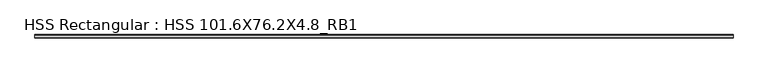
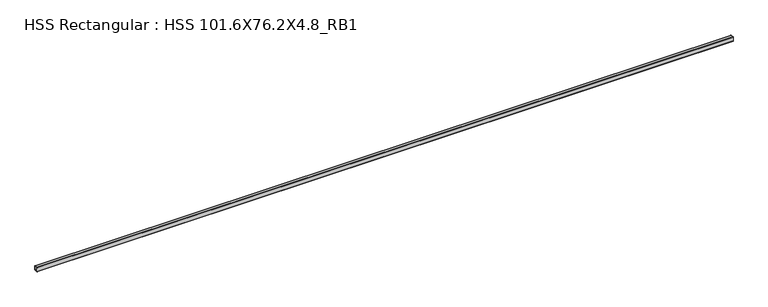
"""IFC4 building model written with IfcOpenShell, lengths in millimetres: beam geometry, HSS Rectangular : HSS 101.6X76.2X4.8_RB1."""

from ifc_helpers import new_model, si_unit, point, frame, frame_2d, origin, place, context, project, spatial, polyline, circle_curve, trimmed, segment, composite_curve, outline, extrude, source, transform, mapped, element, save


def hss_rectangular_hss_101_6x76_2x4_8_rb1_f7a6f8b3(model_context):
    return source(origin(), model_context, "Body", "SweptSolid", [
        extrude(outline(composite_curve([segment(trimmed(circle_curve(frame_2d((-28.575, 41.275)), 9.525), [point((-38.1, 41.275))], [point((-28.575, 50.8))], False, "CARTESIAN"), True, "CONTINUOUS"), segment(polyline([(-28.575, 50.8), (28.575, 50.8)]), True, "CONTINUOUS"), segment(trimmed(circle_curve(frame_2d((28.575, 41.275)), 9.525), [point((28.575, 50.8))], [point((38.1, 41.275))], False, "CARTESIAN"), True, "CONTINUOUS"), segment(polyline([(38.1, 41.275), (38.1, -41.275)]), True, "CONTINUOUS"), segment(trimmed(circle_curve(frame_2d((28.575, -41.275)), 9.525), [point((38.1, -41.275))], [point((28.575, -50.8))], False, "CARTESIAN"), True, "CONTINUOUS"), segment(polyline([(28.575, -50.8), (-28.575, -50.8)]), True, "CONTINUOUS"), segment(trimmed(circle_curve(frame_2d((-28.575, -41.275)), 9.525), [point((-28.575, -50.8))], [point((-38.1, -41.275))], False, "CARTESIAN"), True, "CONTINUOUS"), segment(polyline([(-38.1, -41.275), (-38.1, 41.275)]), True, "CONTINUOUS")], self_intersect=False), holes=[composite_curve([segment(polyline([(28.575, 46.0375), (-28.575, 46.0375)]), True, "CONTINUOUS"), segment(trimmed(circle_curve(frame_2d((-28.575, 41.275)), 4.7625), [point((-28.575, 46.0375))], [point((-33.3375, 41.275))], True, "CARTESIAN"), True, "CONTINUOUS"), segment(polyline([(-33.3375, 41.275), (-33.3375, -41.275)]), True, "CONTINUOUS"), segment(trimmed(circle_curve(frame_2d((-28.575, -41.275)), 4.7625), [point((-33.3375, -41.275))], [point((-28.575, -46.0375))], True, "CARTESIAN"), True, "CONTINUOUS"), segment(polyline([(-28.575, -46.0375), (28.575, -46.0375)]), True, "CONTINUOUS"), segment(trimmed(circle_curve(frame_2d((28.575, -41.275)), 4.7625), [point((28.575, -46.0375))], [point((33.3375, -41.275))], True, "CARTESIAN"), True, "CONTINUOUS"), segment(polyline([(33.3375, -41.275), (33.3375, 41.275)]), True, "CONTINUOUS"), segment(trimmed(circle_curve(frame_2d((28.575, 41.275)), 4.7625), [point((33.3375, 41.275))], [point((28.575, 46.0375))], True, "CARTESIAN"), True, "CONTINUOUS")], self_intersect=False)]), frame((-8985.5753948, 0.0, 0.0), z_axis=(1.0, 0.0, 0.0), x_axis=(0.0, 1.0, 0.0)), (0.0, 0.0, 1.0), 14984.8179793),
    ])


if __name__ == "__main__":
    model = new_model("IFC4")
    model_context = context("Model", 3, world=origin())
    ifc_project = project(units=[si_unit("LENGTHUNIT", "METRE", prefix="MILLI")], contexts=[model_context])
    site = spatial("IfcSite", under=ifc_project)
    building = spatial("IfcBuilding", under=site)
    placement = place(None, origin())
    hss_rectangular_hss_101_6x76_2x4_8_rb1_shape = hss_rectangular_hss_101_6x76_2x4_8_rb1_f7a6f8b3(model_context)
    element("IfcBeam", 1, ObjectType="HSS Rectangular : HSS 101.6X76.2X4.8_RB1", at=placement, inside=building, context=model_context, shape_type="MappedRepresentation", body=[
        mapped(hss_rectangular_hss_101_6x76_2x4_8_rb1_shape, transform((0.0, 0.0, 0.0), x_axis=(1.0, 0.0, 0.0), y_axis=(0.0, 1.0, 0.0), z_axis=(0.0, 0.0, 1.0))),
    ])
    save(model, "model.ifc")

# Revit data of these elements
# Type "HSS Rectangular : HSS 101.6X76.2X4.8_RB1"
#   Section Name Key = "HSS 4X3X3/16"
#   Assembly Code = "B10"
#   Width = 7.62 cm
#   Wall Nominal Thickness = 0.4763 cm
#   Wall Design Thickness = 0.442 cm
#   Torsional Moment of Inertia = 260.561 cm⁴
#   Torsional Modulus = 61.2876 cm³
#   Section Area = 14.4516 cm²
#   Plastic Modulus weak axis = 40.3122 cm³
#   Plastic Modulus strong axis = 49.1612 cm³
#   Perimeter = 0.881482 m²/m
#   Outer Fillet = 0.9525 cm
#   Nominal Weight = 12.1285 kgf/m
#   Moment of Inertia weak axis = 131.529 cm⁴
#   Moment of Inertia strong axis = 205.202 cm⁴
#   Inner Fillet = 0.4763 cm
#   Height = 10.16 cm
#   Elastic Modulus weak axis = 34.4128 cm³
#   Elastic Modulus strong axis = 40.476 cm³
#   Centroid Vertical = 5.08 cm
#   Centroid Horizontal = 3.81 cm
#   Length [instance default] = 1524 mm
#   Structural Material [instance default] = Steel ASTM A500, Grade B, Rectangular and Square
#   Principal Axes Angle = 0
# Element 1 (IfcBeam, "HSS Rectangular : HSS 101.6X76.2X4.8_RB1")
#   Structural Material = Steel ASTM A992
#   Materials on its faces: "Steel ASTM A992"
# Materials
#   "Steel ASTM A500, Grade B, Rectangular and Square": class "Metal", colour RGB 199 199 199, transparency 0, Description = "Carbon steel", Cost = 0
#   "Steel ASTM A992": class "Metal", colour RGB 199 199 199, transparency 0, Description = "Structural steel 50ksi", Cost = 0
